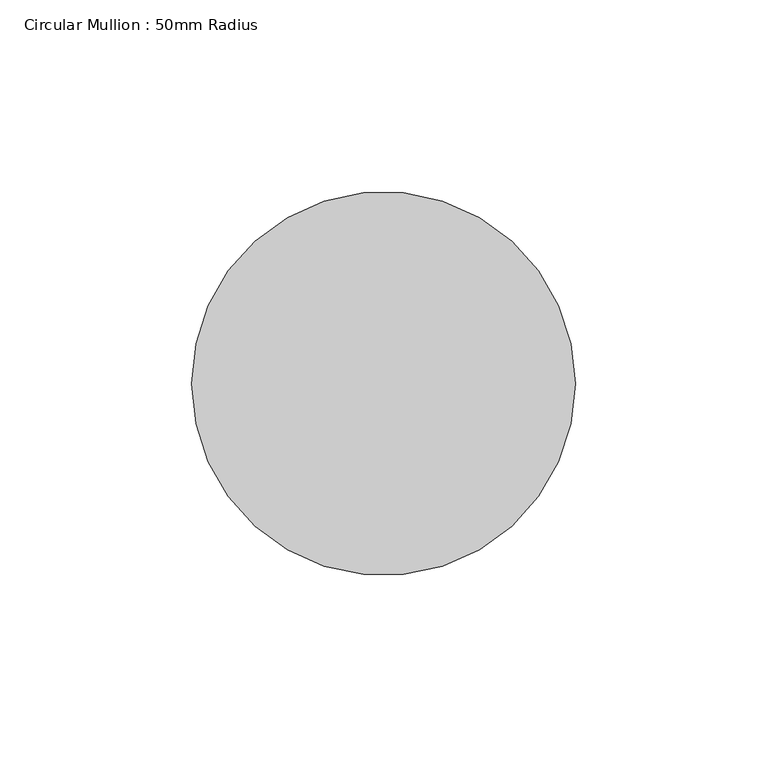
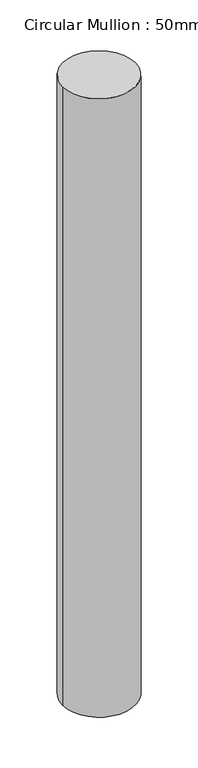
"""IFC4 building model written with IfcOpenShell, lengths in millimetres: member geometry, Circular Mullion : 50mm Radius."""

from ifc_helpers import new_model, si_unit, point, frame, origin, origin_2d, place, context, project, spatial, circle_curve, trimmed, segment, composite_curve, outline, extrude, source, transform, mapped, element, save


def circular_mullion_50mm_radius_dfaaf16f(model_context):
    return source(origin(), model_context, "Body", "SweptSolid", [
        extrude(outline(composite_curve([segment(trimmed(circle_curve(origin_2d(), 50.0), [point((50.0, 0.0))], [point((-50.0, 0.0))], False, "CARTESIAN"), True, "CONTINUOUS"), segment(trimmed(circle_curve(origin_2d(), 50.0), [point((-50.0, 0.0))], [point((50.0, 0.0))], False, "CARTESIAN"), True, "CONTINUOUS")], self_intersect=False)), frame((0.0, 0.0, -900.3944541), z_axis=(0.0, 0.0, 1.0), x_axis=(1.0, 0.0, 0.0)), (0.0, 0.0, 1.0), 900.3944541),
    ])


if __name__ == "__main__":
    model = new_model("IFC4")
    model_context = context("Model", 3, world=origin())
    ifc_project = project(units=[si_unit("LENGTHUNIT", "METRE", prefix="MILLI")], contexts=[model_context])
    site = spatial("IfcSite", under=ifc_project)
    building = spatial("IfcBuilding", under=site)
    placement = place(None, origin())
    circular_mullion_50mm_radius_shape = circular_mullion_50mm_radius_dfaaf16f(model_context)
    element("IfcMember", 1, ObjectType="Circular Mullion : 50mm Radius", at=placement, inside=building, context=model_context, shape_type="MappedRepresentation", body=[
        mapped(circular_mullion_50mm_radius_shape, transform((0.0, 0.0, 0.0), x_axis=(1.0, 0.0, 0.0), y_axis=(0.0, 1.0, 0.0), z_axis=(0.0, 0.0, 1.0))),
    ])
    save(model, "model.ifc")

# Revit data of these elements
# Type "Circular Mullion : 50mm Radius"
#   built-in parameter 1007350 = 0.164042 (stored number, unit not read)
# Element 1 (IfcMember, "Circular Mullion : 50mm Radius")
#   Materials on its faces: "Aluminium"
# Materials
#   "Aluminium": class "Metal", colour RGB 247 247 247, transparency 0, Description = "Aluminium 6061", Cost = 0
